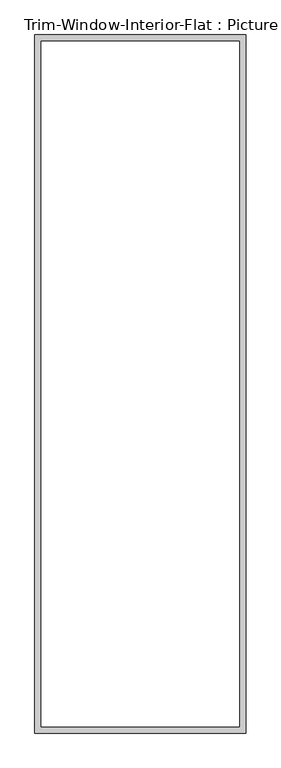
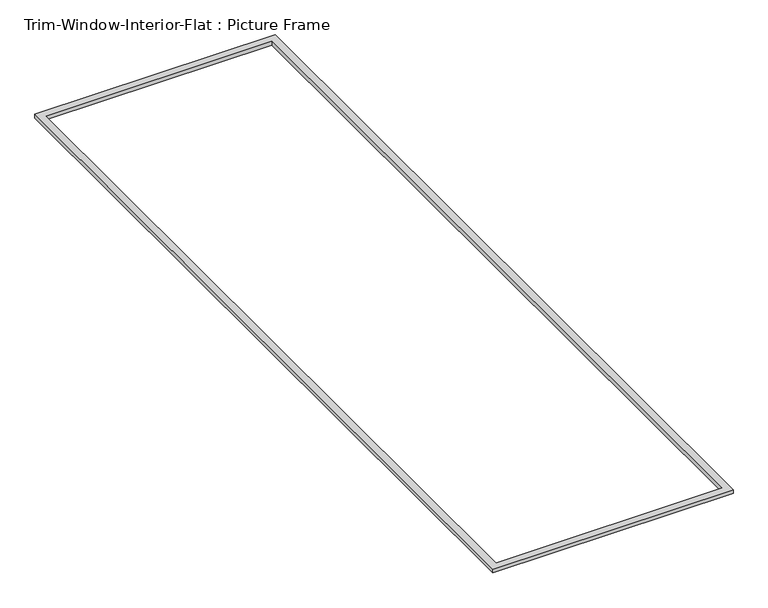
"""IFC4 building model written with IfcOpenShell, lengths in millimetres: proxy geometry, Trim-Window-Interior-Flat : Picture Frame."""

from ifc_helpers import new_model, si_unit, origin, origin_with_axes, place, context, project, spatial, polyline, outline, extrude, source, transform, mapped, element, save


def trim_window_interior_flat_picture_frame_4e25f6c2(model_context):
    return source(origin(), model_context, "Body", "SweptSolid", [
        extrude(outline(polyline([(958.85, 44.45), (958.85, -6292.85), (-958.85, -6292.85), (-958.85, 44.45), (958.85, 44.45)]), holes=[polyline([(901.7, -12.7), (-901.7, -12.7), (-901.7, -6235.7), (901.7, -6235.7), (901.7, -12.7)])]), origin_with_axes(), (0.0, 0.0, 1.0), 31.75),
    ])


if __name__ == "__main__":
    model = new_model("IFC4")
    model_context = context("Model", 3, world=origin())
    ifc_project = project(units=[si_unit("LENGTHUNIT", "METRE", prefix="MILLI")], contexts=[model_context])
    site = spatial("IfcSite", under=ifc_project)
    building = spatial("IfcBuilding", under=site)
    placement = place(None, origin())
    trim_window_interior_flat_picture_frame_shape = trim_window_interior_flat_picture_frame_4e25f6c2(model_context)
    element("IfcBuildingElementProxy", 1, Name="Trim-Window-Interior-Flat : Picture Frame", ObjectType="Trim-Window-Interior-Flat : Picture Frame", at=placement, inside=building, context=model_context, shape_type="MappedRepresentation", body=[
        mapped(trim_window_interior_flat_picture_frame_shape, transform((0.0, 0.0, 0.0), x_axis=(1.0, 0.0, 0.0), y_axis=(0.0, 1.0, 0.0), z_axis=(0.0, 0.0, 1.0))),
    ])
    save(model, "model.ifc")

# Revit data of these elements
# Type "Trim-Window-Interior-Flat : Picture Frame"
#   Trim Thickness_Picture Frame = 0' - 1 1/4"
#   Trim Width = 0' - 2 1/4"
#   Trim Thickness_with Sill = 0' - 0 3/4"
#   Sill Thickness = 0' - 1 1/4"
#   Opening Width [instance default] = 2' - 0"
#   Opening Height [instance default] = 3' - 0"
#   Default Elevation = 4' - 0"
#   Sill = no
#   Picture Frame = yes
#   Trim Material [instance default] = none
# Element 1 (IfcBuildingElementProxy, "Trim-Window-Interior-Flat : Picture Frame")
#   Opening Width = 6' - 0"
#   Opening Height = 20' - 6"
#   Trim Material = Wood - Stained
#   Materials on its faces: "Wood - Stained"
# Materials
#   "Wood - Stained": class "Wood", colour RGB 224 178 126, transparency 0, Cost = 0
